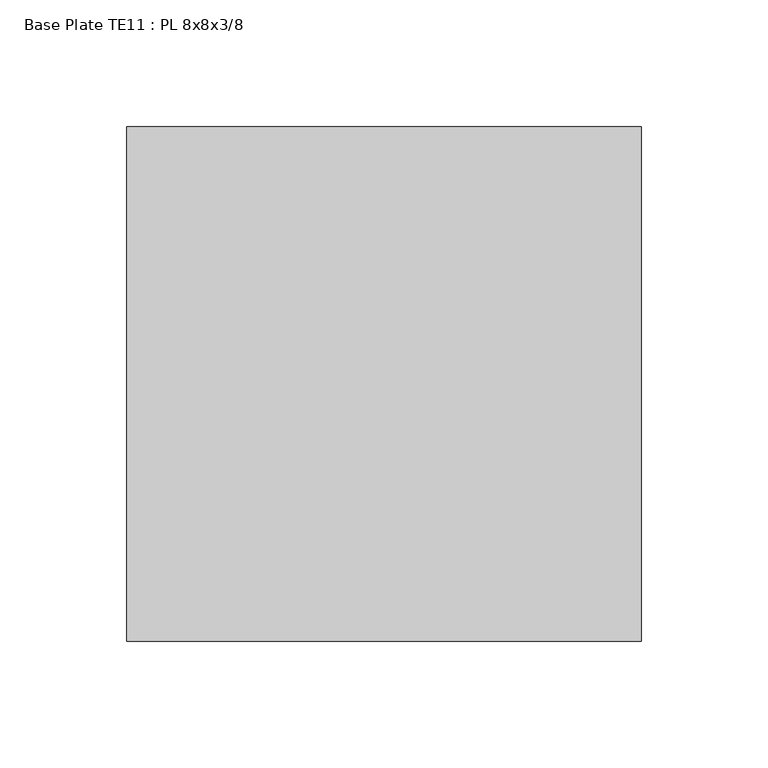
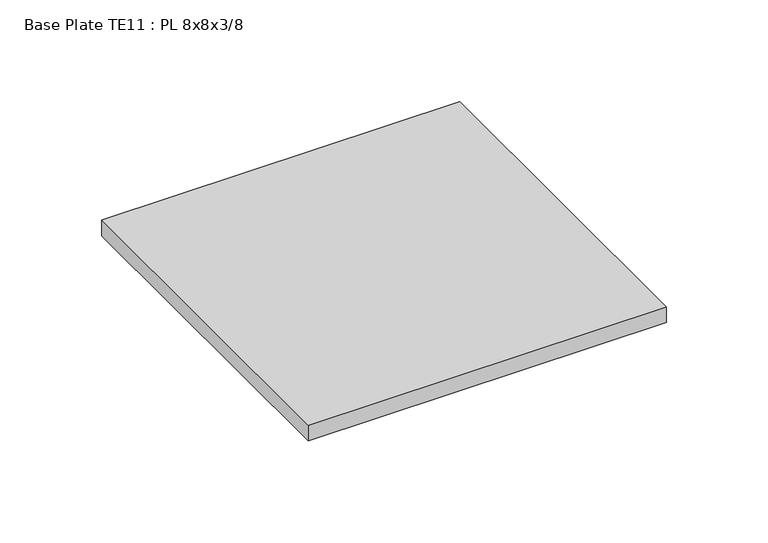
"""IFC4 building model written with IfcOpenShell, lengths in millimetres: proxy geometry, Base Plate TE11 : PL 8x8x3/8."""

from ifc_helpers import new_model, si_unit, frame, origin, place, context, project, spatial, polyline, outline, extrude, source, transform, mapped, element, save


def base_plate_te11_pl_8x8x3_8_a4684d66(model_context):
    return source(origin(), model_context, "Body", "SweptSolid", [
        extrude(outline(polyline([(590318.6599233, -533941.0913841), (590318.6599233, -534144.2913841), (590115.4599233, -534144.2913841), (590115.4599233, -533941.0913841), (590318.6599233, -533941.0913841)])), frame((0.0, 0.0, 19.05), z_axis=(0.0, 0.0, 1.0), x_axis=(1.0, 0.0, 0.0)), (0.0, 0.0, 1.0), 9.525),
    ])


if __name__ == "__main__":
    model = new_model("IFC4")
    model_context = context("Model", 3, world=origin())
    ifc_project = project(units=[si_unit("LENGTHUNIT", "METRE", prefix="MILLI")], contexts=[model_context])
    site = spatial("IfcSite", under=ifc_project)
    building = spatial("IfcBuilding", under=site)
    placement = place(None, origin())
    base_plate_te11_pl_8x8x3_8_shape = base_plate_te11_pl_8x8x3_8_a4684d66(model_context)
    element("IfcBuildingElementProxy", 1, Name="Base Plate TE11 : PL 8x8x3/8", ObjectType="Base Plate TE11 : PL 8x8x3/8", at=placement, inside=building, context=model_context, shape_type="MappedRepresentation", body=[
        mapped(base_plate_te11_pl_8x8x3_8_shape, transform((0.0, 0.0, 0.0), x_axis=(1.0, 0.0, 0.0), y_axis=(0.0, 1.0, 0.0), z_axis=(0.0, 0.0, 1.0))),
    ])
    save(model, "model.ifc")

# Revit data of these elements
# Element 1 (IfcBuildingElementProxy, "Base Plate TE11 : PL 8x8x3/8")
#   Materials on its faces: "GALV. STL BASE PLATE"
# Materials
#   "GALV. STL BASE PLATE": class "Generic", colour RGB 211 211 207, transparency 0, Cost = 0
